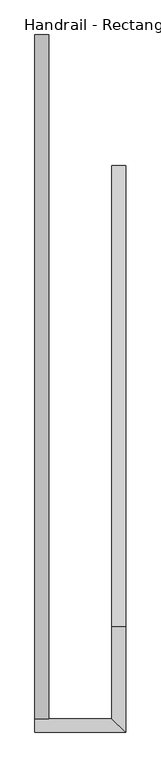
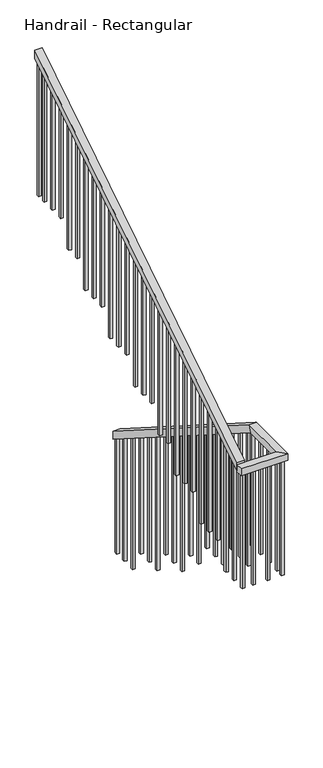
"""IFC4 building model written with IfcOpenShell, lengths in millimetres: railing geometry, Handrail - Rectangular."""

from ifc_helpers import new_model, si_unit, frame, origin, place, context, project, spatial, polyline, outline, extrude, faceted_brep, source, transform, mapped, element, save


def handrail_rectangular_e0900e7e(model_context):
    return source(origin(), model_context, "Body", "SolidModel", [
        faceted_brep([(-74523.6, 12128.5, 20345.4), (-74472.8, 12128.5, 20345.4), (-74472.8, 12128.5, 20285.186276), (-74523.6, 12128.5, 20285.186276), (-74523.6, 10452.1, 21412.2), (-74472.8, 10452.1, 21412.2), (-74472.8, 10437.3070051, 21361.4), (-74523.6, 10437.3070051, 21361.4), (-74523.6, 10115.55, 21412.2), (-74472.8, 10064.75, 21412.2), (-74472.8, 10064.75, 21361.4), (-74523.6, 10115.55, 21361.4), (-74803.0, 10115.55, 21412.2), (-74803.0, 10115.55, 21361.4), (-74803.0, 10064.75, 21361.4), (-74803.0, 10064.75, 21412.2)], [[[0, 1, 2, 3]], [[1, 0, 4, 5]], [[2, 1, 5, 6]], [[3, 2, 6, 7]], [[0, 3, 7, 4]], [[5, 4, 8, 9]], [[6, 5, 9, 10]], [[7, 6, 10, 11]], [[4, 7, 11, 8]], [[12, 13, 14, 15]], [[9, 8, 12, 15]], [[10, 9, 15, 14]], [[11, 10, 14, 13]], [[8, 11, 13, 12]]]),
        faceted_brep([(-74752.2, 10115.55, 21428.3636364), (-74803.0, 10115.55, 21428.3636364), (-74803.0, 10115.55, 21368.1499123), (-74752.2, 10115.55, 21368.1499123), (-74752.2, 12604.75, 23012.4), (-74752.2, 12604.75, 22952.186276), (-74803.0, 12604.75, 22952.186276), (-74803.0, 12604.75, 23012.4)], [[[0, 1, 2, 3]], [[4, 5, 6, 7]], [[1, 0, 4, 7]], [[2, 1, 7, 6]], [[3, 2, 6, 5]], [[0, 3, 5, 4]]]),
        extrude(outline(polyline([(12519.025, 22897.6340032), (12538.075, 22909.7567305), (12538.075, 21920.2), (12519.025, 21920.2), (12519.025, 22897.6340032)])), frame((-74787.125, 0.0, 0.0), z_axis=(1.0, 0.0, 0.0), x_axis=(0.0, 1.0, 0.0)), (0.0, 0.0, 1.0), 19.05),
        extrude(outline(polyline([(12417.425, 22832.9794578), (12436.475, 22845.1021851), (12436.475, 21920.2), (12417.425, 21920.2), (12417.425, 22832.9794578)])), frame((-74787.125, 0.0, 0.0), z_axis=(1.0, 0.0, 0.0), x_axis=(0.0, 1.0, 0.0)), (0.0, 0.0, 1.0), 19.05),
        extrude(outline(polyline([(12315.825, 22768.3249123), (12334.875, 22780.4476396), (12334.875, 21920.2), (12315.825, 21920.2), (12315.825, 22768.3249123)])), frame((-74787.125, 0.0, 0.0), z_axis=(1.0, 0.0, 0.0), x_axis=(0.0, 1.0, 0.0)), (0.0, 0.0, 1.0), 19.05),
        extrude(outline(polyline([(12214.225, 22703.6703669), (12233.275, 22715.7930941), (12233.275, 21742.4), (12214.225, 21742.4), (12214.225, 22703.6703669)])), frame((-74787.125, 0.0, 0.0), z_axis=(1.0, 0.0, 0.0), x_axis=(0.0, 1.0, 0.0)), (0.0, 0.0, 1.0), 19.05),
        extrude(outline(polyline([(12112.625, 22639.0158214), (12131.675, 22651.1385487), (12131.675, 21742.4), (12112.625, 21742.4), (12112.625, 22639.0158214)])), frame((-74787.125, 0.0, 0.0), z_axis=(1.0, 0.0, 0.0), x_axis=(0.0, 1.0, 0.0)), (0.0, 0.0, 1.0), 19.05),
        extrude(outline(polyline([(12011.025, 22574.361276), (12030.075, 22586.4840032), (12030.075, 21564.6), (12011.025, 21564.6), (12011.025, 22574.361276)])), frame((-74787.125, 0.0, 0.0), z_axis=(1.0, 0.0, 0.0), x_axis=(0.0, 1.0, 0.0)), (0.0, 0.0, 1.0), 19.05),
        extrude(outline(polyline([(11909.425, 22509.7067305), (11928.475, 22521.8294578), (11928.475, 21564.6), (11909.425, 21564.6), (11909.425, 22509.7067305)])), frame((-74787.125, 0.0, 0.0), z_axis=(1.0, 0.0, 0.0), x_axis=(0.0, 1.0, 0.0)), (0.0, 0.0, 1.0), 19.05),
        extrude(outline(polyline([(11807.825, 22445.0521851), (11826.875, 22457.1749123), (11826.875, 21564.6), (11807.825, 21564.6), (11807.825, 22445.0521851)])), frame((-74787.125, 0.0, 0.0), z_axis=(1.0, 0.0, 0.0), x_axis=(0.0, 1.0, 0.0)), (0.0, 0.0, 1.0), 19.05),
        extrude(outline(polyline([(11706.225, 22380.3976396), (11725.275, 22392.5203669), (11725.275, 21386.8), (11706.225, 21386.8), (11706.225, 22380.3976396)])), frame((-74787.125, 0.0, 0.0), z_axis=(1.0, 0.0, 0.0), x_axis=(0.0, 1.0, 0.0)), (0.0, 0.0, 1.0), 19.05),
        extrude(outline(polyline([(11604.625, 22315.7430941), (11623.675, 22327.8658214), (11623.675, 21386.8), (11604.625, 21386.8), (11604.625, 22315.7430941)])), frame((-74787.125, 0.0, 0.0), z_axis=(1.0, 0.0, 0.0), x_axis=(0.0, 1.0, 0.0)), (0.0, 0.0, 1.0), 19.05),
        extrude(outline(polyline([(11503.025, 22251.0885487), (11522.075, 22263.211276), (11522.075, 21386.8), (11503.025, 21386.8), (11503.025, 22251.0885487)])), frame((-74787.125, 0.0, 0.0), z_axis=(1.0, 0.0, 0.0), x_axis=(0.0, 1.0, 0.0)), (0.0, 0.0, 1.0), 19.05),
        extrude(outline(polyline([(11401.425, 22186.4340032), (11420.475, 22198.5567305), (11420.475, 21209.0), (11401.425, 21209.0), (11401.425, 22186.4340032)])), frame((-74787.125, 0.0, 0.0), z_axis=(1.0, 0.0, 0.0), x_axis=(0.0, 1.0, 0.0)), (0.0, 0.0, 1.0), 19.05),
        extrude(outline(polyline([(11299.825, 22121.7794578), (11318.875, 22133.9021851), (11318.875, 21209.0), (11299.825, 21209.0), (11299.825, 22121.7794578)])), frame((-74787.125, 0.0, 0.0), z_axis=(1.0, 0.0, 0.0), x_axis=(0.0, 1.0, 0.0)), (0.0, 0.0, 1.0), 19.05),
        extrude(outline(polyline([(11198.225, 22057.1249123), (11217.275, 22069.2476396), (11217.275, 21209.0), (11198.225, 21209.0), (11198.225, 22057.1249123)])), frame((-74787.125, 0.0, 0.0), z_axis=(1.0, 0.0, 0.0), x_axis=(0.0, 1.0, 0.0)), (0.0, 0.0, 1.0), 19.05),
        extrude(outline(polyline([(11096.625, 21992.4703669), (11115.675, 22004.5930941), (11115.675, 21031.2), (11096.625, 21031.2), (11096.625, 21992.4703669)])), frame((-74787.125, 0.0, 0.0), z_axis=(1.0, 0.0, 0.0), x_axis=(0.0, 1.0, 0.0)), (0.0, 0.0, 1.0), 19.05),
        extrude(outline(polyline([(10995.025, 21927.8158214), (11014.075, 21939.9385487), (11014.075, 21031.2), (10995.025, 21031.2), (10995.025, 21927.8158214)])), frame((-74787.125, 0.0, 0.0), z_axis=(1.0, 0.0, 0.0), x_axis=(0.0, 1.0, 0.0)), (0.0, 0.0, 1.0), 19.05),
        extrude(outline(polyline([(10893.425, 21863.161276), (10912.475, 21875.2840032), (10912.475, 20853.4), (10893.425, 20853.4), (10893.425, 21863.161276)])), frame((-74787.125, 0.0, 0.0), z_axis=(1.0, 0.0, 0.0), x_axis=(0.0, 1.0, 0.0)), (0.0, 0.0, 1.0), 19.05),
        extrude(outline(polyline([(10791.825, 21798.5067305), (10810.875, 21810.6294578), (10810.875, 20853.4), (10791.825, 20853.4), (10791.825, 21798.5067305)])), frame((-74787.125, 0.0, 0.0), z_axis=(1.0, 0.0, 0.0), x_axis=(0.0, 1.0, 0.0)), (0.0, 0.0, 1.0), 19.05),
        extrude(outline(polyline([(10690.225, 21733.8521851), (10709.275, 21745.9749123), (10709.275, 20853.4), (10690.225, 20853.4), (10690.225, 21733.8521851)])), frame((-74787.125, 0.0, 0.0), z_axis=(1.0, 0.0, 0.0), x_axis=(0.0, 1.0, 0.0)), (0.0, 0.0, 1.0), 19.05),
        extrude(outline(polyline([(10588.625, 21669.1976396), (10607.675, 21681.3203669), (10607.675, 20675.6), (10588.625, 20675.6), (10588.625, 21669.1976396)])), frame((-74787.125, 0.0, 0.0), z_axis=(1.0, 0.0, 0.0), x_axis=(0.0, 1.0, 0.0)), (0.0, 0.0, 1.0), 19.05),
        extrude(outline(polyline([(10487.025, 21604.5430941), (10506.075, 21616.6658214), (10506.075, 20675.6), (10487.025, 20675.6), (10487.025, 21604.5430941)])), frame((-74787.125, 0.0, 0.0), z_axis=(1.0, 0.0, 0.0), x_axis=(0.0, 1.0, 0.0)), (0.0, 0.0, 1.0), 19.05),
        extrude(outline(polyline([(10385.425, 21539.8885487), (10404.475, 21552.011276), (10404.475, 20675.6), (10385.425, 20675.6), (10385.425, 21539.8885487)])), frame((-74787.125, 0.0, 0.0), z_axis=(1.0, 0.0, 0.0), x_axis=(0.0, 1.0, 0.0)), (0.0, 0.0, 1.0), 19.05),
        extrude(outline(polyline([(10283.825, 21475.2340032), (10302.875, 21487.3567305), (10302.875, 20497.8), (10283.825, 20497.8), (10283.825, 21475.2340032)])), frame((-74787.125, 0.0, 0.0), z_axis=(1.0, 0.0, 0.0), x_axis=(0.0, 1.0, 0.0)), (0.0, 0.0, 1.0), 19.05),
        extrude(outline(polyline([(10182.225, 21410.5794578), (10201.275, 21422.7021851), (10201.275, 20497.8), (10182.225, 20497.8), (10182.225, 21410.5794578)])), frame((-74787.125, 0.0, 0.0), z_axis=(1.0, 0.0, 0.0), x_axis=(0.0, 1.0, 0.0)), (0.0, 0.0, 1.0), 19.05),
        extrude(outline(polyline([(-74691.875, 10099.675), (-74691.875, 10080.625), (-74710.925, 10080.625), (-74710.925, 10099.675), (-74691.875, 10099.675)])), frame((0.0, 0.0, 20497.8), z_axis=(0.0, 0.0, 1.0), x_axis=(1.0, 0.0, 0.0)), (0.0, 0.0, 1.0), 863.6),
        extrude(outline(polyline([(-74590.275, 10099.675), (-74590.275, 10080.625), (-74609.325, 10080.625), (-74609.325, 10099.675), (-74590.275, 10099.675)])), frame((0.0, 0.0, 20497.8), z_axis=(0.0, 0.0, 1.0), x_axis=(1.0, 0.0, 0.0)), (0.0, 0.0, 1.0), 863.6),
        extrude(outline(polyline([(-74507.725, 10156.825), (-74488.675, 10156.825), (-74488.675, 10137.775), (-74507.725, 10137.775), (-74507.725, 10156.825)])), frame((0.0, 0.0, 20497.8), z_axis=(0.0, 0.0, 1.0), x_axis=(1.0, 0.0, 0.0)), (0.0, 0.0, 1.0), 863.6),
        extrude(outline(polyline([(-74507.725, 10258.425), (-74488.675, 10258.425), (-74488.675, 10239.375), (-74507.725, 10239.375), (-74507.725, 10258.425)])), frame((0.0, 0.0, 20497.8), z_axis=(0.0, 0.0, 1.0), x_axis=(1.0, 0.0, 0.0)), (0.0, 0.0, 1.0), 863.6),
        extrude(outline(polyline([(-74507.725, 10360.025), (-74488.675, 10360.025), (-74488.675, 10340.975), (-74507.725, 10340.975), (-74507.725, 10360.025)])), frame((0.0, 0.0, 20497.8), z_axis=(0.0, 0.0, 1.0), x_axis=(1.0, 0.0, 0.0)), (0.0, 0.0, 1.0), 863.6),
        extrude(outline(polyline([(10493.375, 21325.7203669), (10512.425, 21313.5976396), (10512.425, 20320.0), (10493.375, 20320.0), (10493.375, 21325.7203669)])), frame((-74507.725, 0.0, 0.0), z_axis=(1.0, 0.0, 0.0), x_axis=(0.0, 1.0, 0.0)), (0.0, 0.0, 1.0), 19.05),
        extrude(outline(polyline([(10594.975, 21261.0658214), (10614.025, 21248.9430941), (10614.025, 20320.0), (10594.975, 20320.0), (10594.975, 21261.0658214)])), frame((-74507.725, 0.0, 0.0), z_axis=(1.0, 0.0, 0.0), x_axis=(0.0, 1.0, 0.0)), (0.0, 0.0, 1.0), 19.05),
        extrude(outline(polyline([(10696.575, 21196.411276), (10715.625, 21184.2885487), (10715.625, 20320.0), (10696.575, 20320.0), (10696.575, 21196.411276)])), frame((-74507.725, 0.0, 0.0), z_axis=(1.0, 0.0, 0.0), x_axis=(0.0, 1.0, 0.0)), (0.0, 0.0, 1.0), 19.05),
        extrude(outline(polyline([(10798.175, 21131.7567305), (10817.225, 21119.6340032), (10817.225, 20142.2), (10798.175, 20142.2), (10798.175, 21131.7567305)])), frame((-74507.725, 0.0, 0.0), z_axis=(1.0, 0.0, 0.0), x_axis=(0.0, 1.0, 0.0)), (0.0, 0.0, 1.0), 19.05),
        extrude(outline(polyline([(10899.775, 21067.1021851), (10918.825, 21054.9794578), (10918.825, 20142.2), (10899.775, 20142.2), (10899.775, 21067.1021851)])), frame((-74507.725, 0.0, 0.0), z_axis=(1.0, 0.0, 0.0), x_axis=(0.0, 1.0, 0.0)), (0.0, 0.0, 1.0), 19.05),
        extrude(outline(polyline([(11001.375, 21002.4476396), (11020.425, 20990.3249123), (11020.425, 20142.2), (11001.375, 20142.2), (11001.375, 21002.4476396)])), frame((-74507.725, 0.0, 0.0), z_axis=(1.0, 0.0, 0.0), x_axis=(0.0, 1.0, 0.0)), (0.0, 0.0, 1.0), 19.05),
        extrude(outline(polyline([(11102.975, 20937.7930941), (11122.025, 20925.6703669), (11122.025, 19964.4), (11102.975, 19964.4), (11102.975, 20937.7930941)])), frame((-74507.725, 0.0, 0.0), z_axis=(1.0, 0.0, 0.0), x_axis=(0.0, 1.0, 0.0)), (0.0, 0.0, 1.0), 19.05),
        extrude(outline(polyline([(11204.575, 20873.1385487), (11223.625, 20861.0158214), (11223.625, 19964.4), (11204.575, 19964.4), (11204.575, 20873.1385487)])), frame((-74507.725, 0.0, 0.0), z_axis=(1.0, 0.0, 0.0), x_axis=(0.0, 1.0, 0.0)), (0.0, 0.0, 1.0), 19.05),
        extrude(outline(polyline([(11306.175, 20808.4840032), (11325.225, 20796.361276), (11325.225, 19786.6), (11306.175, 19786.6), (11306.175, 20808.4840032)])), frame((-74507.725, 0.0, 0.0), z_axis=(1.0, 0.0, 0.0), x_axis=(0.0, 1.0, 0.0)), (0.0, 0.0, 1.0), 19.05),
        extrude(outline(polyline([(11407.775, 20743.8294578), (11426.825, 20731.7067305), (11426.825, 19786.6), (11407.775, 19786.6), (11407.775, 20743.8294578)])), frame((-74507.725, 0.0, 0.0), z_axis=(1.0, 0.0, 0.0), x_axis=(0.0, 1.0, 0.0)), (0.0, 0.0, 1.0), 19.05),
        extrude(outline(polyline([(11509.375, 20679.1749123), (11528.425, 20667.0521851), (11528.425, 19786.6), (11509.375, 19786.6), (11509.375, 20679.1749123)])), frame((-74507.725, 0.0, 0.0), z_axis=(1.0, 0.0, 0.0), x_axis=(0.0, 1.0, 0.0)), (0.0, 0.0, 1.0), 19.05),
        extrude(outline(polyline([(11610.975, 20614.5203669), (11630.025, 20602.3976396), (11630.025, 19608.8), (11610.975, 19608.8), (11610.975, 20614.5203669)])), frame((-74507.725, 0.0, 0.0), z_axis=(1.0, 0.0, 0.0), x_axis=(0.0, 1.0, 0.0)), (0.0, 0.0, 1.0), 19.05),
        extrude(outline(polyline([(11712.575, 20549.8658214), (11731.625, 20537.7430941), (11731.625, 19608.8), (11712.575, 19608.8), (11712.575, 20549.8658214)])), frame((-74507.725, 0.0, 0.0), z_axis=(1.0, 0.0, 0.0), x_axis=(0.0, 1.0, 0.0)), (0.0, 0.0, 1.0), 19.05),
        extrude(outline(polyline([(11814.175, 20485.211276), (11833.225, 20473.0885487), (11833.225, 19608.8), (11814.175, 19608.8), (11814.175, 20485.211276)])), frame((-74507.725, 0.0, 0.0), z_axis=(1.0, 0.0, 0.0), x_axis=(0.0, 1.0, 0.0)), (0.0, 0.0, 1.0), 19.05),
        extrude(outline(polyline([(11915.775, 20420.5567305), (11934.825, 20408.4340032), (11934.825, 19431.0), (11915.775, 19431.0), (11915.775, 20420.5567305)])), frame((-74507.725, 0.0, 0.0), z_axis=(1.0, 0.0, 0.0), x_axis=(0.0, 1.0, 0.0)), (0.0, 0.0, 1.0), 19.05),
        extrude(outline(polyline([(12017.375, 20355.9021851), (12036.425, 20343.7794578), (12036.425, 19431.0), (12017.375, 19431.0), (12017.375, 20355.9021851)])), frame((-74507.725, 0.0, 0.0), z_axis=(1.0, 0.0, 0.0), x_axis=(0.0, 1.0, 0.0)), (0.0, 0.0, 1.0), 19.05),
        extrude(outline(polyline([(-74768.075, 10099.675), (-74768.075, 10080.625), (-74787.125, 10080.625), (-74787.125, 10099.675), (-74768.075, 10099.675)])), frame((0.0, 0.0, 20497.8), z_axis=(0.0, 0.0, 1.0), x_axis=(1.0, 0.0, 0.0)), (0.0, 0.0, 1.0), 863.6),
        extrude(outline(polyline([(-74507.725, 10099.675), (-74488.675, 10099.675), (-74488.675, 10080.625), (-74507.725, 10080.625), (-74507.725, 10099.675)])), frame((0.0, 0.0, 20497.8), z_axis=(0.0, 0.0, 1.0), x_axis=(1.0, 0.0, 0.0)), (0.0, 0.0, 1.0), 863.6),
        extrude(outline(polyline([(10442.575, 21358.0476396), (10461.625, 21345.9249123), (10461.625, 20497.8), (10442.575, 20497.8), (10442.575, 21358.0476396)])), frame((-74507.725, 0.0, 0.0), z_axis=(1.0, 0.0, 0.0), x_axis=(0.0, 1.0, 0.0)), (0.0, 0.0, 1.0), 19.05),
        extrude(outline(polyline([(12585.7, 22940.0635487), (12604.75, 22952.186276), (12604.75, 21920.2), (12585.7, 21920.2), (12585.7, 22940.0635487)])), frame((-74787.125, 0.0, 0.0), z_axis=(1.0, 0.0, 0.0), x_axis=(0.0, 1.0, 0.0)), (0.0, 0.0, 1.0), 19.05),
        extrude(outline(polyline([(12109.45, 20297.3090032), (12128.5, 20285.186276), (12128.5, 19431.0), (12109.45, 19431.0), (12109.45, 20297.3090032)])), frame((-74507.725, 0.0, 0.0), z_axis=(1.0, 0.0, 0.0), x_axis=(0.0, 1.0, 0.0)), (0.0, 0.0, 1.0), 19.05),
    ])


if __name__ == "__main__":
    model = new_model("IFC4")
    model_context = context("Model", 3, world=origin())
    ifc_project = project(units=[si_unit("LENGTHUNIT", "METRE", prefix="MILLI")], contexts=[model_context])
    site = spatial("IfcSite", under=ifc_project)
    building = spatial("IfcBuilding", under=site)
    placement = place(None, origin())
    handrail_rectangular_shape = handrail_rectangular_e0900e7e(model_context)
    element("IfcRailing", 1, ObjectType="Handrail - Rectangular", at=placement, inside=building, context=model_context, shape_type="MappedRepresentation", body=[
        mapped(handrail_rectangular_shape, transform((0.0, 0.0, 0.0), x_axis=(1.0, 0.0, 0.0), y_axis=(0.0, 1.0, 0.0), z_axis=(0.0, 0.0, 1.0))),
    ])
    save(model, "model.ifc")
